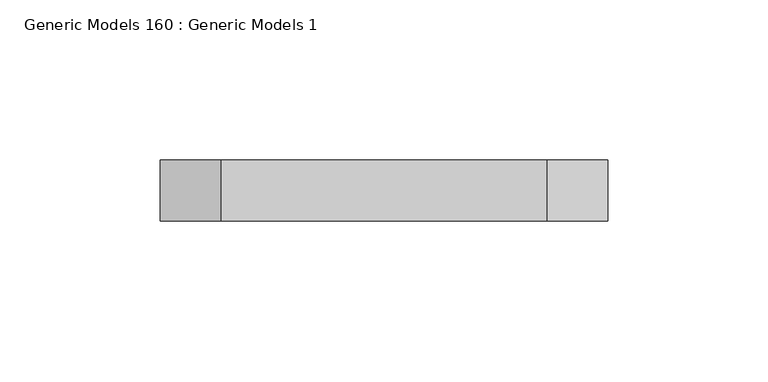
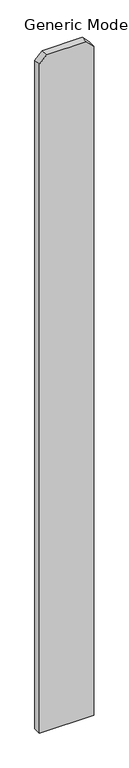
"""IFC4 building model written with IfcOpenShell, lengths in millimetres: proxy geometry, Generic Models 160 : Generic Models 1."""

from ifc_helpers import new_model, si_unit, frame, origin, place, context, project, spatial, polyline, outline, extrude, source, transform, mapped, element, save


def generic_models_160_generic_models_1_9801a194(model_context):
    return source(origin(), model_context, "Body", "SweptSolid", [
        extrude(outline(polyline([(76.2, 54379.8125), (1885.95, 54379.8125), (1905.0, 54360.7625), (1905.0, 54259.1625), (1885.95, 54240.1125), (76.2, 54240.1125), (76.2, 54379.8125)])), frame((0.0, 547.6875, 0.0), z_axis=(0.0, 1.0, 0.0), x_axis=(0.0, 0.0, 1.0)), (0.0, 0.0, 1.0), 19.05),
    ])


if __name__ == "__main__":
    model = new_model("IFC4")
    model_context = context("Model", 3, world=origin())
    ifc_project = project(units=[si_unit("LENGTHUNIT", "METRE", prefix="MILLI")], contexts=[model_context])
    site = spatial("IfcSite", under=ifc_project)
    building = spatial("IfcBuilding", under=site)
    placement = place(None, origin())
    generic_models_160_generic_models_1_shape = generic_models_160_generic_models_1_9801a194(model_context)
    element("IfcBuildingElementProxy", 1, Name="Generic Models 160 : Generic Models 1", ObjectType="Generic Models 160 : Generic Models 1", at=placement, inside=building, context=model_context, shape_type="MappedRepresentation", body=[
        mapped(generic_models_160_generic_models_1_shape, transform((0.0, 0.0, 0.0), x_axis=(1.0, 0.0, 0.0), y_axis=(0.0, 1.0, 0.0), z_axis=(0.0, 0.0, 1.0))),
    ])
    save(model, "model.ifc")

# Revit data of these elements
# Element 1 (IfcBuildingElementProxy, "Generic Models 160 : Generic Models 1")
#   Materials on its faces: "VERTICAL 1X6 CEDAR PLANKS W/ CLEAR WOOD SEALER"
# Materials
#   "VERTICAL 1X6 CEDAR PLANKS W/ CLEAR WOOD SEALER": class "Wood", colour RGB 234 198 147, transparency 0, Description = "Pinus Echinata", Cost = 0
